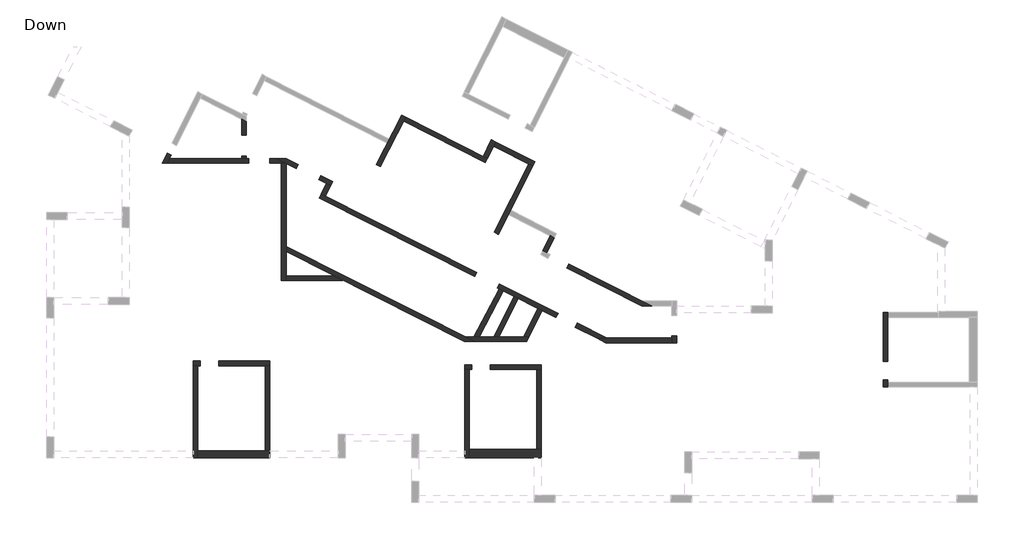
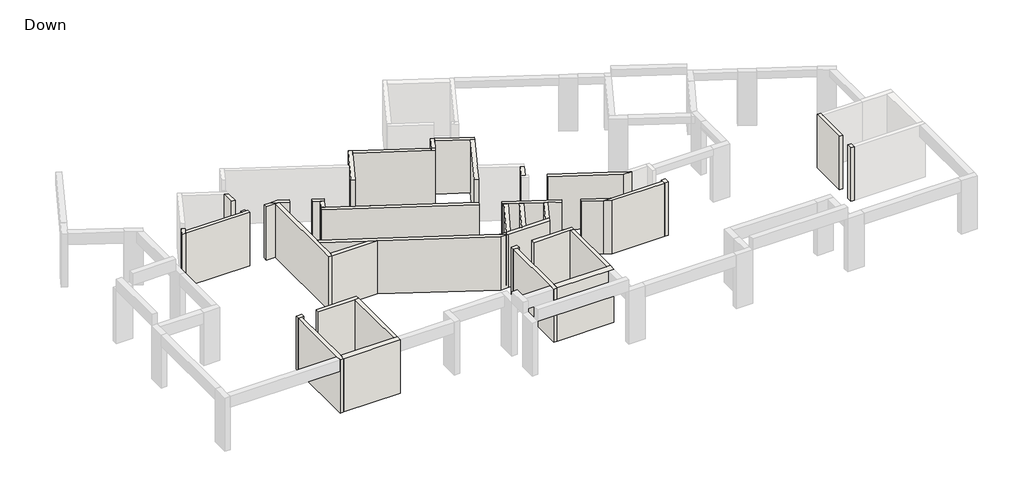
# One storey, part 1 of 3: 39 walls.
"""IFC4 building model written with IfcOpenShell, lengths in millimetres."""

from ifc_helpers import new_model, si_unit, origin, origin_with_axes, place, context, project, spatial, polyline, outline, extrude, faceted_brep, element, save

model = new_model("IFC4")

# Units and contexts
model_context = context("Model", 3, world=origin())
ifc_project = project(units=[si_unit("LENGTHUNIT", "METRE", prefix="MILLI")], contexts=[model_context])

# Site, building, storey
site = spatial("IfcSite", under=ifc_project)
building = spatial("IfcBuilding", under=site)
storey = spatial("IfcBuildingStorey", under=building, Name="Down", Elevation=0.0)

# Walls
placement = place(None, origin())
element("IfcWall", 1, ObjectType="20", at=placement, inside=storey, context=model_context, shape_type="Brep", body=[
    faceted_brep([(-10046.1154665, -6780.8119163, 0.0), (-10046.1154665, -6580.8119163, 0.0), (-10046.1154665, -5543.6743788, 0.0), (-10046.1154665, -5319.6317102, 0.0), (-10046.1154665, -1741.3845051, 0.0), (-10046.1154665, -1741.3845051, 3080.0), (-10046.1154665, -5319.6317102, 3080.0), (-10046.1154665, -5543.6743788, 3080.0), (-10046.1154665, -6580.8119163, 3080.0), (-10046.1154665, -6780.8119163, 3080.0), (-10246.1154665, -6780.8119163, 0.0), (-10246.1154665, -6780.8119163, 2780.0), (-10246.1154665, -6780.8119163, 3080.0), (-10246.1154665, -1726.4993482, 3080.0), (-10246.1154665, -1726.4993482, 2780.0), (-10246.1154665, -1726.4993482, 0.0), (-10075.8857802, -1726.4993482, 0.0), (-10075.8857802, -1726.4993482, 3080.0)], [[[0, 1, 2, 3, 4, 5, 6, 7, 8, 9]], [[10, 11, 12, 13, 14, 15]], [[4, 3, 2, 1, 0, 10, 15, 16]], [[9, 8, 7, 6, 5, 17, 13, 12]], [[5, 4, 16, 17]], [[16, 15, 14, 13, 17]], [[0, 9, 12, 11, 10]]]),
])
element("IfcWall", 2, ObjectType="20", at=placement, inside=storey, context=model_context, shape_type="Brep", body=[
    faceted_brep([(-10475.8857802, -1526.4993482, 0.0), (-10748.7939096, -1526.4993482, 0.0), (-10748.7939096, -1526.4993482, 2780.0), (-10748.7939096, -1526.4993482, 3080.0), (-10475.8857802, -1526.4993482, 3080.0), (-10075.8857802, -1726.4993482, 0.0), (-10075.8857802, -1726.4993482, 3080.0), (-10246.1154665, -1726.4993482, 3080.0), (-10748.7939096, -1726.4993482, 3080.0), (-10748.7939096, -1726.4993482, 2780.0), (-10748.7939096, -1726.4993482, 0.0), (-10246.1154665, -1726.4993482, 0.0)], [[[0, 1, 2, 3, 4]], [[5, 6, 7, 8, 9, 10, 11]], [[1, 0, 5, 11, 10]], [[3, 2, 1, 10, 9, 8]], [[4, 3, 8, 7, 6]], [[0, 4, 6, 5]]]),
])
element("IfcWall", 3, ObjectType="20", at=placement, inside=storey, context=model_context, shape_type="Brep", body=[
    faceted_brep([(-11648.323755, -1526.4993482, 0.0), (-11760.5135249, -1526.4993482, 0.0), (-11960.5135249, -1526.4993482, 0.0), (-15053.2787931, -1526.4993482, 0.0), (-15053.2787931, -1526.4993482, 2780.0), (-15053.2787931, -1526.4993482, 3080.0), (-11960.5135249, -1526.4993482, 3080.0), (-11760.5135249, -1526.4993482, 3080.0), (-11648.323755, -1526.4993482, 3080.0), (-11648.323755, -1526.4993482, 2780.0), (-11648.323755, -1726.4993482, 0.0), (-11648.323755, -1726.4993482, 2780.0), (-11648.323755, -1726.4993482, 3080.0), (-15153.2787931, -1726.4993482, 3080.0), (-15153.2787931, -1726.4993482, 0.0)], [[[0, 1, 2, 3, 4, 5, 6, 7, 8, 9]], [[10, 11, 12, 13, 14]], [[3, 2, 1, 0, 10, 14]], [[8, 7, 6, 5, 13, 12]], [[0, 9, 8, 12, 11, 10]], [[5, 4, 3, 14, 13]]]),
])
element("IfcWall", 4, ObjectType="20", at=placement, inside=storey, context=model_context, shape_type="Brep", body=[
    faceted_brep([(-15153.2787931, -1726.4993482, 0.0), (-15053.2787931, -1526.4993482, 0.0), (-14980.4135975, -1380.768957, 0.0), (-14980.4135975, -1380.768957, 2780.0), (-14980.4135975, -1380.768957, 3080.0), (-15053.2787931, -1526.4993482, 3080.0), (-15153.2787931, -1726.4993482, 3080.0), (-15376.8855909, -1726.4993482, 0.0), (-15376.8855909, -1726.4993482, 2780.0), (-15376.8855909, -1726.4993482, 3080.0), (-15159.2990357, -1291.3262379, 3080.0), (-15159.2990357, -1291.3262379, 2780.0), (-15159.2990357, -1291.3262379, 0.0)], [[[0, 1, 2, 3, 4, 5, 6]], [[7, 8, 9, 10, 11, 12]], [[2, 1, 0, 7, 12]], [[4, 3, 2, 12, 11, 10]], [[6, 5, 4, 10, 9]], [[0, 6, 9, 8, 7]]]),
])
element("IfcWall", 5, ObjectType="20", at=placement, inside=storey, context=model_context, shape_type="Brep", body=[
    faceted_brep([(-11960.5135249, 170.863779, 0.0), (-11960.5135249, -518.38158, 0.0), (-11960.5135249, -518.38158, 2780.0), (-11960.5135249, -518.38158, 3080.0), (-11960.5135249, 170.863779, 3080.0), (-11960.5135249, 170.863779, 2780.0), (-11760.5135249, 69.5479895, 0.0), (-11760.5135249, 69.5479895, 3080.0), (-11760.5135249, -518.38158, 3080.0), (-11760.5135249, -518.38158, 2780.0), (-11760.5135249, -518.38158, 0.0)], [[[0, 1, 2, 3, 4, 5]], [[6, 7, 8, 9, 10]], [[1, 0, 6, 10]], [[3, 2, 1, 10, 9, 8]], [[4, 3, 8, 7]], [[0, 5, 4, 7, 6]]]),
])
element("IfcWall", 6, ObjectType="20", at=placement, inside=storey, context=model_context, shape_type="Brep", body=[
    faceted_brep([(-11960.5135249, -1425.9636596, 0.0), (-11960.5135249, -1526.4993482, 0.0), (-11960.5135249, -1526.4993482, 2780.0), (-11960.5135249, -1526.4993482, 3080.0), (-11960.5135249, -1425.9636596, 3080.0), (-11960.5135249, -1425.9636596, 2780.0), (-11760.5135249, -1425.9636596, 0.0), (-11760.5135249, -1425.9636596, 2780.0), (-11760.5135249, -1425.9636596, 3080.0), (-11760.5135249, -1526.4993482, 3080.0), (-11760.5135249, -1526.4993482, 2780.0), (-11760.5135249, -1526.4993482, 0.0)], [[[0, 1, 2, 3, 4, 5]], [[6, 7, 8, 9, 10, 11]], [[1, 0, 6, 11]], [[4, 3, 9, 8]], [[0, 5, 4, 8, 7, 6]], [[3, 2, 1, 11, 10, 9]]]),
])
element("IfcWall", 7, ObjectType="20", at=placement, inside=storey, context=model_context, shape_type="Brep", body=[
    faceted_brep([(-5982.9078517, -1881.7028715, 0.0), (-4985.9127135, 79.4194333, 0.0), (-4895.2767918, 257.7032792, 0.0), (-4895.2767918, 257.7032792, 3080.0), (-4985.9127135, 79.4194333, 3080.0), (-5982.9078517, -1881.7028715, 3080.0), (-6161.1916976, -1791.0669498, 0.0), (-6161.1916976, -1791.0669498, 2780.0), (-6161.1916976, -1791.0669498, 3080.0), (-5688.8111915, -861.8789214, 3080.0), (-5598.1752698, -683.5950755, 3080.0), (-5073.5606377, 348.3392009, 3080.0), (-5073.5606377, 348.3392009, 2780.0), (-5073.5606377, 348.3392009, 0.0), (-5598.1752698, -683.5950755, 0.0), (-5688.8111915, -861.8789214, 0.0)], [[[0, 1, 2, 3, 4, 5]], [[6, 7, 8, 9, 10, 11, 12, 13, 14, 15]], [[2, 1, 0, 6, 15, 14, 13]], [[5, 4, 3, 11, 10, 9, 8]], [[0, 5, 8, 7, 6]], [[3, 2, 13, 12, 11]]]),
])
element("IfcWall", 8, ObjectType="20", at=placement, inside=storey, context=model_context, shape_type="Brep", body=[
    faceted_brep([(-4985.9127135, 79.4194333, 0.0), (-1478.212729, -1703.8246929, 0.0), (-1478.212729, -1703.8246929, 3080.0), (-4985.9127135, 79.4194333, 3080.0), (-4895.2767918, 257.7032792, 0.0), (-4895.2767918, 257.7032792, 3080.0), (-1565.8606533, -1434.9049253, 3080.0), (-1387.5768074, -1525.540847, 3080.0), (-1387.5768074, -1525.540847, 0.0), (-1565.8606533, -1434.9049253, 0.0)], [[[0, 1, 2, 3]], [[4, 5, 6, 7, 8, 9]], [[1, 0, 4, 9, 8]], [[3, 2, 7, 6, 5]], [[0, 3, 5, 4]], [[2, 1, 8, 7]]]),
])
element("IfcWall", 9, ObjectType="20", at=placement, inside=storey, context=model_context, shape_type="Brep", body=[
    faceted_brep([(-1387.5768074, -1525.540847, 0.0), (-1115.669538, -990.6902841, 0.0), (-1025.0331208, -812.4054634, 0.0), (-1025.0331208, -812.4054634, 3080.0), (-1115.669538, -990.6902841, 3080.0), (-1387.5768074, -1525.540847, 3080.0), (-1565.8606533, -1434.9049253, 0.0), (-1565.8606533, -1434.9049253, 2780.0), (-1565.8606533, -1434.9049253, 3080.0), (-1203.6166871, -722.3591018, 3080.0), (-1203.6166871, -722.3591018, 2780.0), (-1203.6166871, -722.3591018, 0.0)], [[[0, 1, 2, 3, 4, 5]], [[6, 7, 8, 9, 10, 11]], [[2, 1, 0, 6, 11]], [[5, 4, 3, 9, 8]], [[0, 5, 8, 7, 6]], [[3, 2, 11, 10, 9]]]),
])
element("IfcWall", 10, ObjectType="20", at=placement, inside=storey, context=model_context, shape_type="Brep", body=[
    faceted_brep([(-1115.669538, -990.6902841, 0.0), (402.8730243, -1756.3779423, 0.0), (581.4556142, -1846.4238115, 0.0), (581.4556142, -1846.4238115, 3080.0), (402.8730243, -1756.3779423, 3080.0), (-1115.669538, -990.6902841, 3080.0), (-1025.0331208, -812.4054634, 0.0), (-1025.0331208, -812.4054634, 3080.0), (54.7682985, -1356.8687143, 3080.0), (671.5014835, -1667.8412216, 3080.0), (671.5014835, -1667.8412216, 2780.0), (671.5014835, -1667.8412216, 0.0)], [[[0, 1, 2, 3, 4, 5]], [[6, 7, 8, 9, 10, 11]], [[2, 1, 0, 6, 11]], [[5, 4, 3, 9, 8, 7]], [[0, 5, 7, 6]], [[3, 2, 11, 10, 9]]]),
])
element("IfcWall", 11, ObjectType="20", at=placement, inside=storey, context=model_context, shape_type="Brep", body=[
    faceted_brep([(402.8730243, -1756.3779423, 0.0), (-1082.8838189, -4702.990676, 0.0), (-1082.8838189, -4702.990676, 3080.0), (402.8730243, -1756.3779423, 3080.0), (581.4556142, -1846.4238115, 0.0), (581.4556142, -1846.4238115, 3080.0), (-382.0351871, -3757.2575237, 3080.0), (-472.0818656, -3935.8417186, 3080.0), (-904.301229, -4793.0365453, 3080.0), (-904.301229, -4793.0365453, 2780.0), (-904.301229, -4793.0365453, 0.0), (-472.0818656, -3935.8417186, 0.0), (-382.0351871, -3757.2575237, 0.0)], [[[0, 1, 2, 3]], [[4, 5, 6, 7, 8, 9, 10, 11, 12]], [[1, 0, 4, 12, 11, 10]], [[2, 1, 10, 9, 8]], [[3, 2, 8, 7, 6, 5]], [[0, 3, 5, 4]]]),
])
element("IfcWall", 12, ObjectType="20", at=placement, inside=storey, context=model_context, shape_type="Brep", body=[
    faceted_brep([(1327.1276693, -4852.636386, 0.0), (1001.0372857, -5493.9474736, 0.0), (1001.0372857, -5493.9474736, 3080.0), (1327.1276693, -4852.636386, 3080.0), (1327.1276693, -4852.636386, 2780.0), (1505.3269714, -4943.4385782, 0.0), (1505.3269714, -4943.4385782, 3080.0), (1179.5082357, -5584.2154251, 3080.0), (1179.5082357, -5584.2154251, 2780.0), (1179.5082357, -5584.2154251, 0.0)], [[[0, 1, 2, 3, 4]], [[5, 6, 7, 8, 9]], [[1, 0, 5, 9]], [[3, 2, 7, 6]], [[0, 4, 3, 6, 5]], [[2, 1, 9, 8, 7]]]),
])
element("IfcWall", 13, ObjectType="20", at=placement, inside=storey, context=model_context, shape_type="Brep", body=[
    faceted_brep([(2035.1126004, -6241.094009, 0.0), (5265.429403, -7874.9401934, 0.0), (5265.429403, -7874.9401934, 2780.0), (5265.429403, -7874.9401934, 3080.0), (2035.1126004, -6241.094009, 3080.0), (2035.1126004, -6241.094009, 2780.0), (2125.3803454, -6062.6234674, 0.0), (2125.3803454, -6062.6234674, 2780.0), (2125.3803454, -6062.6234674, 3080.0), (5313.1307352, -7674.9401934, 3080.0), (5708.5555718, -7874.9401934, 3080.0), (5708.5555718, -7874.9401934, 0.0), (5313.1307352, -7674.9401934, 0.0), (2077.6096629, -6157.072039, 3080.0)], [[[0, 1, 2, 3, 4, 5]], [[6, 7, 8, 9, 10, 11, 12]], [[1, 0, 6, 12, 11]], [[4, 3, 10, 9, 8, 13]], [[0, 5, 4, 13, 8, 7, 6]], [[3, 2, 1, 11, 10]]]),
])
element("IfcWall", 14, ObjectType="20", at=placement, inside=storey, context=model_context, shape_type="Brep", body=[
    faceted_brep([(6570.8726693, -9167.2116828, 0.0), (6570.8726693, -9268.8187486, 0.0), (6570.8726693, -9468.8187486, 0.0), (6570.8726693, -9468.8187486, 3080.0), (6570.8726693, -9268.8187486, 3080.0), (6570.8726693, -9167.2116828, 3080.0), (6570.8726693, -9167.2116828, 2780.0), (6770.8726693, -9167.2116828, 0.0), (6770.8726693, -9167.2116828, 2780.0), (6770.8726693, -9167.2116828, 3080.0), (6770.8726693, -9468.8187486, 3080.0), (6770.8726693, -9468.8187486, 2780.0), (6770.8726693, -9468.8187486, 0.0)], [[[0, 1, 2, 3, 4, 5, 6]], [[7, 8, 9, 10, 11, 12]], [[2, 1, 0, 7, 12]], [[5, 4, 3, 10, 9]], [[0, 6, 5, 9, 8, 7]], [[3, 2, 12, 11, 10]]]),
])
element("IfcWall", 15, ObjectType="20", at=placement, inside=storey, context=model_context, shape_type="Brep", body=[
    faceted_brep([(6570.8726693, -9268.8187486, 0.0), (3765.4759744, -9268.8187486, 0.0), (3322.4500467, -9268.8187486, 0.0), (3322.4500467, -9268.8187486, 3080.0), (3765.4759744, -9268.8187486, 3080.0), (6570.8726693, -9268.8187486, 3080.0), (6570.8726693, -9268.8187486, 2780.0), (6570.8726693, -9468.8187486, 0.0), (6570.8726693, -9468.8187486, 3080.0), (3717.7625467, -9468.8187486, 3080.0), (3717.7625467, -9468.8187486, 2780.0), (3717.7625467, -9468.8187486, 0.0)], [[[0, 1, 2, 3, 4, 5, 6]], [[7, 8, 9, 10, 11]], [[2, 1, 0, 7, 11]], [[5, 4, 3, 9, 8]], [[0, 6, 5, 8, 7]], [[3, 2, 11, 10, 9]]]),
])
element("IfcWall", 16, ObjectType="20", at=placement, inside=storey, context=model_context, shape_type="Brep", body=[
    faceted_brep([(3765.4759744, -9268.8187486, 0.0), (2487.4451637, -8622.2260855, 0.0), (2487.4451637, -8622.2260855, 2780.0), (2487.4451637, -8622.2260855, 3080.0), (3765.4759744, -9268.8187486, 3080.0), (3765.4759744, -9268.8187486, 2780.0), (3322.4500467, -9268.8187486, 0.0), (3322.4500467, -9268.8187486, 3080.0), (2397.1569943, -8800.6862953, 3080.0), (2397.1569943, -8800.6862953, 2780.0), (2397.1569943, -8800.6862953, 0.0)], [[[0, 1, 2, 3, 4, 5]], [[6, 7, 8, 9, 10]], [[1, 0, 6, 10]], [[3, 2, 1, 10, 9, 8]], [[4, 3, 8, 7]], [[0, 5, 4, 7, 6]]]),
])
element("IfcWall", 17, ObjectType="20", at=placement, inside=storey, context=model_context, shape_type="Brep", body=[
    faceted_brep([(1666.9910125, -8207.1346573, 0.0), (-860.136602, -6928.58788, 0.0), (-860.136602, -6928.58788, 2780.0), (-860.136602, -6928.58788, 3080.0), (1666.9910125, -8207.1346573, 3080.0), (1666.9910125, -8207.1346573, 2780.0), (1576.7028432, -8385.594867, 0.0), (1576.7028432, -8385.594867, 2780.0), (1576.7028432, -8385.594867, 3080.0), (979.8740908, -8083.6419805, 3080.0), (979.5487996, -8083.4774063, 3080.0), (801.086592, -7993.1882261, 3080.0), (-42.8153908, -7566.2338633, 3080.0), (-221.2756006, -7475.9456939, 3080.0), (-696.8020222, -7235.3631565, 3080.0), (-875.2761926, -7145.067924, 3080.0), (-950.4247713, -7107.0480897, 3080.0), (-950.4247713, -7107.0480897, 2780.0), (-950.4247713, -7107.0480897, 0.0), (-875.2761926, -7145.067924, 0.0), (-696.8020222, -7235.3631565, 0.0), (-221.2756006, -7475.9456939, 0.0), (-42.8153908, -7566.2338633, 0.0), (801.086592, -7993.1882261, 0.0), (979.5487996, -8083.4774063, 0.0)], [[[0, 1, 2, 3, 4, 5]], [[6, 7, 8, 9, 10, 11, 12, 13, 14, 15, 16, 17, 18, 19, 20, 21, 22, 23, 24]], [[1, 0, 6, 24, 23, 22, 21, 20, 19, 18]], [[3, 2, 1, 18, 17, 16]], [[4, 3, 16, 15, 14, 13, 12, 11, 10, 9, 8]], [[0, 5, 4, 8, 7, 6]]]),
])
element("IfcWall", 18, ObjectType="20", at=placement, inside=storey, context=model_context, shape_type="Brep", body=[
    faceted_brep([(-1838.1570872, -6436.8740342, 0.0), (-8353.2474072, -3147.7022221, 0.0), (-8531.7861682, -3057.5661486, 0.0), (-8531.7861682, -3057.5661486, 3080.0), (-8353.2474072, -3147.7022221, 3080.0), (-1838.1570872, -6436.8740342, 3080.0), (-1838.1570872, -6436.8740342, 2780.0), (-1928.2924837, -6615.4114541, 0.0), (-1928.2924837, -6615.4114541, 3080.0), (-8621.2295591, -3236.4529305, 3080.0), (-8621.2295591, -3236.4529305, 0.0), (-1927.470094, -6613.7824899, 3080.0)], [[[0, 1, 2, 3, 4, 5, 6]], [[7, 8, 9, 10]], [[2, 1, 0, 7, 10]], [[5, 4, 3, 9, 8, 11]], [[0, 6, 5, 11, 8, 7]], [[3, 2, 10, 9]]]),
])
element("IfcWall", 19, ObjectType="20", at=placement, inside=storey, context=model_context, shape_type="Brep", body=[
    faceted_brep([(-8353.2474072, -3147.7022221, 0.0), (-8129.2939322, -2699.7952722, 0.0), (-8129.2939322, -2699.7952722, 3080.0), (-8353.2474072, -3147.7022221, 3080.0), (-8353.2474072, -3147.7022221, 2780.0), (-8531.7861682, -3057.5661486, 0.0), (-8531.7861682, -3057.5661486, 3080.0), (-8308.1793704, -2610.3525531, 3080.0), (-8308.1793704, -2610.3525531, 0.0)], [[[0, 1, 2, 3, 4]], [[5, 6, 7, 8]], [[1, 0, 5, 8]], [[3, 2, 7, 6]], [[0, 4, 3, 6, 5]], [[2, 1, 8, 7]]]),
])
element("IfcWall", 20, ObjectType="20", at=placement, inside=storey, context=model_context, shape_type="Brep", body=[
    faceted_brep([(-8039.8512131, -2520.909834, 0.0), (-8558.6189839, -2261.5259486, 0.0), (-8558.6189839, -2261.5259486, 2780.0), (-8558.6189839, -2261.5259486, 3080.0), (-8039.8512131, -2520.909834, 3080.0), (-8039.8512131, -2520.909834, 2780.0), (-8129.2939322, -2699.7952722, 0.0), (-8129.2939322, -2699.7952722, 3080.0), (-8308.1793704, -2610.3525531, 3080.0), (-8648.061703, -2440.4113868, 3080.0), (-8648.061703, -2440.4113868, 2780.0), (-8648.061703, -2440.4113868, 0.0), (-8308.1793704, -2610.3525531, 0.0)], [[[0, 1, 2, 3, 4, 5]], [[6, 7, 8, 9, 10, 11, 12]], [[1, 0, 6, 12, 11]], [[3, 2, 1, 11, 10, 9]], [[4, 3, 9, 8, 7]], [[0, 5, 4, 7, 6]]]),
])
element("IfcWall", 21, ObjectType="20", at=placement, inside=storey, context=model_context, shape_type="Brep", body=[
    faceted_brep([(-9512.4602897, -1784.6052957, 0.0), (-10028.6721847, -1526.4993482, 0.0), (-10028.6721847, -1526.4993482, 2780.0), (-10028.6721847, -1526.4993482, 3080.0), (-9512.4602897, -1784.6052957, 3080.0), (-9512.4602897, -1784.6052957, 2780.0), (-9601.9030088, -1963.4907339, 0.0), (-9601.9030088, -1963.4907339, 2780.0), (-9601.9030088, -1963.4907339, 3080.0), (-10046.1154665, -1741.3845051, 3080.0), (-10075.8857802, -1726.4993482, 3080.0), (-10475.8857802, -1526.4993482, 3080.0), (-10475.8857802, -1526.4993482, 0.0), (-10075.8857802, -1726.4993482, 0.0), (-10046.1154665, -1741.3845051, 0.0)], [[[0, 1, 2, 3, 4, 5]], [[6, 7, 8, 9, 10, 11, 12, 13, 14]], [[1, 0, 6, 14, 13, 12]], [[4, 3, 11, 10, 9, 8]], [[0, 5, 4, 8, 7, 6]], [[3, 2, 1, 12, 11]]]),
])
element("IfcWall", 22, ObjectType="20", at=placement, inside=storey, context=model_context, shape_type="Brep", body=[
    faceted_brep([(-10738.2112055, -10257.2302015, 0.0), (-12939.4136509, -10257.2302015, 0.0), (-12939.4136509, -10257.2302015, 2780.0), (-12939.4136509, -10257.2302015, 3080.0), (-10738.2112055, -10257.2302015, 3080.0), (-10738.2112055, -10257.2302015, 2780.0), (-10738.2112055, -10457.2302015, 0.0), (-10738.2112055, -10457.2302015, 3080.0), (-10938.2112055, -10457.2302015, 3080.0), (-12939.4136509, -10457.2302015, 3080.0), (-12939.4136509, -10457.2302015, 2780.0), (-12939.4136509, -10457.2302015, 0.0), (-10938.2112055, -10457.2302015, 0.0)], [[[0, 1, 2, 3, 4, 5]], [[6, 7, 8, 9, 10, 11, 12]], [[1, 0, 6, 12, 11]], [[3, 2, 1, 11, 10, 9]], [[4, 3, 9, 8, 7]], [[0, 5, 4, 7, 6]]]),
])
element("IfcWall", 23, ObjectType="20", at=placement, inside=storey, context=model_context, shape_type="Brep", body=[
    faceted_brep([(-13738.4078078, -10257.2302015, 0.0), (-14040.0148736, -10257.2302015, 0.0), (-14040.0148736, -10257.2302015, 2780.0), (-14040.0148736, -10257.2302015, 3080.0), (-13738.4078078, -10257.2302015, 3080.0), (-13738.4078078, -10257.2302015, 2780.0), (-13738.4078078, -10457.2302015, 0.0), (-13738.4078078, -10457.2302015, 2780.0), (-13738.4078078, -10457.2302015, 3080.0), (-13840.0148736, -10457.2302015, 3080.0), (-14040.0148736, -10457.2302015, 3080.0), (-14040.0148736, -10457.2302015, 0.0), (-13840.0148736, -10457.2302015, 0.0)], [[[0, 1, 2, 3, 4, 5]], [[6, 7, 8, 9, 10, 11, 12]], [[1, 0, 6, 12, 11]], [[4, 3, 10, 9, 8]], [[0, 5, 4, 8, 7, 6]], [[3, 2, 1, 11, 10]]]),
])
element("IfcWall", 24, ObjectType="20", at=placement, inside=storey, context=model_context, shape_type="Brep", body=[
    faceted_brep([(-14040.0148736, -10457.2302015, 0.0), (-14040.0148736, -14416.2328988, 0.0), (-14040.0148736, -14416.2328988, 3080.0), (-14040.0148736, -14116.2328988, 3080.0), (-14040.0148736, -10457.2302015, 3080.0), (-13840.0148736, -10457.2302015, 0.0), (-13840.0148736, -10457.2302015, 2780.0), (-13840.0148736, -10457.2302015, 3080.0), (-13840.0148736, -14116.2328988, 3080.0), (-13840.0148736, -14416.2328988, 3080.0), (-13840.0148736, -14416.2328988, 0.0), (-13840.0148736, -14116.2328988, 0.0)], [[[0, 1, 2, 3, 4]], [[5, 6, 7, 8, 9, 10, 11]], [[1, 0, 5, 11, 10]], [[4, 3, 2, 9, 8, 7]], [[0, 4, 7, 6, 5]], [[2, 1, 10, 9]]]),
])
element("IfcWall", 25, ObjectType="20", at=placement, inside=storey, context=model_context, shape_type="Brep", body=[
    faceted_brep([(-10738.2112055, -14116.2328988, 0.0), (-10738.2112055, -10457.2302015, 0.0), (-10738.2112055, -10457.2302015, 3080.0), (-10738.2112055, -14116.2328988, 3080.0), (-10738.2112055, -14116.2328988, 2780.0), (-10938.2112055, -14116.2328988, 0.0), (-10938.2112055, -14116.2328988, 2780.0), (-10938.2112055, -14116.2328988, 3080.0), (-10938.2112055, -10457.2302015, 3080.0), (-10938.2112055, -10457.2302015, 2780.0), (-10938.2112055, -10457.2302015, 0.0)], [[[0, 1, 2, 3, 4]], [[5, 6, 7, 8, 9, 10]], [[1, 0, 5, 10]], [[3, 2, 8, 7]], [[0, 4, 3, 7, 6, 5]], [[2, 1, 10, 9, 8]]]),
])
element("IfcWall", 26, ObjectType="20", at=placement, inside=storey, context=model_context, shape_type="Brep", body=[
    faceted_brep([(945.0940817, -10417.0421397, 0.0), (-1256.1083637, -10417.0421397, 0.0), (-1256.1083637, -10417.0421397, 2780.0), (-1256.1083637, -10417.0421397, 3080.0), (945.0940817, -10417.0421397, 3080.0), (945.0940817, -10417.0421397, 2780.0), (945.0940817, -10617.0421397, 0.0), (945.0940817, -10617.0421397, 3080.0), (745.0940817, -10617.0421397, 3080.0), (-1256.1083637, -10617.0421397, 3080.0), (-1256.1083637, -10617.0421397, 2780.0), (-1256.1083637, -10617.0421397, 0.0), (745.0940817, -10617.0421397, 0.0)], [[[0, 1, 2, 3, 4, 5]], [[6, 7, 8, 9, 10, 11, 12]], [[1, 0, 6, 12, 11]], [[3, 2, 1, 11, 10, 9]], [[4, 3, 9, 8, 7]], [[0, 5, 4, 7, 6]]]),
])
element("IfcWall", 27, ObjectType="20", at=placement, inside=storey, context=model_context, shape_type="Brep", body=[
    faceted_brep([(-2055.1025205, -10417.0421397, 0.0), (-2356.7095864, -10417.0421397, 0.0), (-2356.7095864, -10417.0421397, 2780.0), (-2356.7095864, -10417.0421397, 3080.0), (-2055.1025205, -10417.0421397, 3080.0), (-2055.1025205, -10417.0421397, 2780.0), (-2055.1025205, -10617.0421397, 0.0), (-2055.1025205, -10617.0421397, 2780.0), (-2055.1025205, -10617.0421397, 3080.0), (-2156.7095864, -10617.0421397, 3080.0), (-2356.7095864, -10617.0421397, 3080.0), (-2356.7095864, -10617.0421397, 0.0), (-2156.7095864, -10617.0421397, 0.0)], [[[0, 1, 2, 3, 4, 5]], [[6, 7, 8, 9, 10, 11, 12]], [[1, 0, 6, 12, 11]], [[4, 3, 10, 9, 8]], [[0, 5, 4, 8, 7, 6]], [[3, 2, 1, 11, 10]]]),
])
element("IfcWall", 28, ObjectType="20", at=placement, inside=storey, context=model_context, shape_type="Brep", body=[
    faceted_brep([(-2356.7095864, -10617.0421397, 0.0), (-2356.7095864, -14416.2328988, 0.0), (-2356.7095864, -14416.2328988, 2430.0), (-2356.7095864, -14416.2328988, 3080.0), (-2356.7095864, -14116.2328988, 3080.0), (-2356.7095864, -10617.0421397, 3080.0), (-2156.7095864, -10617.0421397, 0.0), (-2156.7095864, -10617.0421397, 2780.0), (-2156.7095864, -10617.0421397, 3080.0), (-2156.7095864, -14066.2328988, 3080.0), (-2156.7095864, -14416.2328988, 3080.0), (-2156.7095864, -14416.2328988, 0.0), (-2156.7095864, -14066.2328988, 0.0)], [[[0, 1, 2, 3, 4, 5]], [[6, 7, 8, 9, 10, 11, 12]], [[1, 0, 6, 12, 11]], [[5, 4, 3, 10, 9, 8]], [[0, 5, 8, 7, 6]], [[3, 2, 1, 11, 10]]]),
])
element("IfcWall", 29, ObjectType="20", at=placement, inside=storey, context=model_context, shape_type="Brep", body=[
    faceted_brep([(945.0940817, -14066.2328988, 0.0), (945.0940817, -10617.0421397, 0.0), (945.0940817, -10617.0421397, 3080.0), (945.0940817, -14066.2328988, 3080.0), (745.0940817, -14066.2328988, 0.0), (745.0940817, -14066.2328988, 2780.0), (745.0940817, -14066.2328988, 3080.0), (745.0940817, -10617.0421397, 3080.0), (745.0940817, -10617.0421397, 2780.0), (745.0940817, -10617.0421397, 0.0)], [[[0, 1, 2, 3]], [[4, 5, 6, 7, 8, 9]], [[1, 0, 4, 9]], [[3, 2, 7, 6]], [[0, 3, 6, 5, 4]], [[2, 1, 9, 8, 7]]]),
])
element("IfcWall", 30, ObjectType="20", at=placement, inside=storey, context=model_context, shape_type="Brep", body=[
    faceted_brep([(15670.9267875, -11066.8070624, 0.0), (15670.9267875, -11368.4141282, 0.0), (15670.9267875, -11368.4141282, 2780.0), (15670.9267875, -11368.4141282, 3080.0), (15670.9267875, -11066.8070624, 3080.0), (15670.9267875, -11066.8070624, 2780.0), (15870.9267875, -11066.8070624, 0.0), (15870.9267875, -11066.8070624, 2780.0), (15870.9267875, -11066.8070624, 3080.0), (15870.9267875, -11168.4141282, 3080.0), (15870.9267875, -11368.4141282, 3080.0), (15870.9267875, -11368.4141282, 0.0), (15870.9267875, -11168.4141282, 0.0)], [[[0, 1, 2, 3, 4, 5]], [[6, 7, 8, 9, 10, 11, 12]], [[1, 0, 6, 12, 11]], [[4, 3, 10, 9, 8]], [[0, 5, 4, 8, 7, 6]], [[3, 2, 1, 11, 10]]]),
])
element("IfcWall", 31, ObjectType="20", at=placement, inside=storey, context=model_context, shape_type="Brep", body=[
    faceted_brep([(15870.9267875, -10267.8129055, 0.0), (15870.9267875, -8367.1461487, 0.0), (15870.9267875, -8167.1461487, 0.0), (15870.9267875, -8167.1461487, 3080.0), (15870.9267875, -8367.1461487, 3080.0), (15870.9267875, -10267.8129055, 3080.0), (15870.9267875, -10267.8129055, 2780.0), (15670.9267875, -10267.8129055, 0.0), (15670.9267875, -10267.8129055, 2780.0), (15670.9267875, -10267.8129055, 3080.0), (15670.9267875, -8167.1461487, 3080.0), (15670.9267875, -8167.1461487, 2780.0), (15670.9267875, -8167.1461487, 0.0)], [[[0, 1, 2, 3, 4, 5, 6]], [[7, 8, 9, 10, 11, 12]], [[2, 1, 0, 7, 12]], [[5, 4, 3, 10, 9]], [[0, 6, 5, 9, 8, 7]], [[3, 2, 12, 11, 10]]]),
])
element("IfcWall", 32, ObjectType="20", at=placement, inside=storey, context=model_context, shape_type="Brep", body=[
    faceted_brep([(-10046.1154665, -6780.8119163, 0.0), (-7595.6314981, -6780.8119163, 0.0), (-7595.6314981, -6780.8119163, 2780.0), (-7595.6314981, -6780.8119163, 3080.0), (-10046.1154665, -6780.8119163, 3080.0), (-7991.7853443, -6580.8119163, 0.0), (-10046.1154665, -6580.8119163, 0.0), (-10046.1154665, -6580.8119163, 3080.0), (-7991.7853443, -6580.8119163, 3080.0)], [[[0, 1, 2, 3, 4]], [[5, 6, 7, 8]], [[1, 0, 6, 5]], [[4, 3, 8, 7]], [[0, 4, 7, 6]], [[3, 2, 1, 5, 8]]]),
])
element("IfcWall", 33, ObjectType="20", at=placement, inside=storey, context=model_context, shape_type="Brep", body=[
    faceted_brep([(-10046.1154665, -5543.6743788, 0.0), (-7991.7853443, -6580.8119163, 0.0), (-7595.6314981, -6780.8119163, 0.0), (-2368.5637573, -9419.7199019, 0.0), (-2368.5637573, -9419.7199019, 2780.0), (-2368.5637573, -9419.7199019, 3080.0), (-7595.6314981, -6780.8119163, 3080.0), (-7991.7853443, -6580.8119163, 3080.0), (-10046.1154665, -5543.6743788, 3080.0), (-1924.7869329, -9419.7199019, 0.0), (-2320.9407791, -9219.7199019, 0.0), (-10046.1154665, -5319.6317102, 0.0), (-10046.1154665, -5319.6317102, 3080.0), (-2320.9407791, -9219.7199019, 3080.0), (-1924.7869329, -9419.7199019, 3080.0)], [[[0, 1, 2, 3, 4, 5, 6, 7, 8]], [[9, 10, 11, 12, 13, 14]], [[3, 2, 1, 0, 11, 10, 9]], [[8, 7, 6, 5, 14, 13, 12]], [[5, 4, 3, 9, 14]], [[0, 8, 12, 11]]]),
])
element("IfcWall", 34, ObjectType="20", at=placement, inside=storey, context=model_context, shape_type="Brep", body=[
    faceted_brep([(-1924.7869329, -9419.7199019, 0.0), (311.4275518, -9419.7199019, 0.0), (311.4275518, -9419.7199019, 2780.0), (311.4275518, -9419.7199019, 3080.0), (-1924.7869329, -9419.7199019, 3080.0), (-2320.9407791, -9219.7199019, 0.0), (-2320.9407791, -9219.7199019, 3080.0), (-1957.7033115, -9219.7199019, 3080.0), (-1732.1185851, -9219.7199019, 3080.0), (-1103.5012868, -9219.7199019, 3080.0), (-879.361687, -9219.7199019, 3080.0), (187.820754, -9219.7199019, 3080.0), (411.4275518, -9219.7199019, 3080.0), (411.4275518, -9219.7199019, 0.0), (187.820754, -9219.7199019, 0.0), (-879.361687, -9219.7199019, 0.0), (-1103.5012868, -9219.7199019, 0.0), (-1732.1185851, -9219.7199019, 0.0), (-1957.7033115, -9219.7199019, 0.0)], [[[0, 1, 2, 3, 4]], [[5, 6, 7, 8, 9, 10, 11, 12, 13, 14, 15, 16, 17, 18]], [[1, 0, 5, 18, 17, 16, 15, 14, 13]], [[4, 3, 12, 11, 10, 9, 8, 7, 6]], [[0, 4, 6, 5]], [[3, 2, 1, 13, 12]]]),
])
element("IfcWall", 35, ObjectType="20", at=placement, inside=storey, context=model_context, shape_type="Brep", body=[
    faceted_brep([(411.4275518, -9219.7199019, 0.0), (979.5487996, -8083.4774063, 0.0), (979.5487996, -8083.4774063, 3080.0), (945.0940817, -8152.386842, 3080.0), (411.4275518, -9219.7199019, 3080.0), (187.820754, -9219.7199019, 0.0), (187.820754, -9219.7199019, 3080.0), (801.086592, -7993.1882261, 3080.0), (801.086592, -7993.1882261, 0.0)], [[[0, 1, 2, 3, 4]], [[5, 6, 7, 8]], [[1, 0, 5, 8]], [[4, 3, 2, 7, 6]], [[0, 4, 6, 5]], [[2, 1, 8, 7]]]),
])
element("IfcWall", 36, ObjectType="20", at=placement, inside=storey, context=model_context, shape_type="SweptSolid", body=[
    extrude(outline(polyline([(-42.8153908, -7566.2338633), (-879.361687, -9219.7199019), (-1103.5012868, -9219.7199019), (-221.2756006, -7475.9456939), (-42.8153908, -7566.2338633)])), origin_with_axes(), (0.0, 0.0, 1.0), 3080.0),
])
element("IfcWall", 37, ObjectType="20", at=placement, inside=storey, context=model_context, shape_type="SweptSolid", body=[
    extrude(outline(polyline([(-696.8020222, -7235.3631565), (-1732.1185851, -9219.7199019), (-1957.7033115, -9219.7199019), (-875.2761926, -7145.067924), (-696.8020222, -7235.3631565)])), origin_with_axes(), (0.0, 0.0, 1.0), 3080.0),
])
element("IfcWall", 38, ObjectType="30", at=placement, inside=storey, context=model_context, shape_type="Brep", body=[
    faceted_brep([(-13840.0148736, -14416.2328988, 0.0), (-10738.2112055, -14416.2328988, 0.0), (-10738.2112055, -14416.2328988, 2430.0), (-10738.2112055, -14416.2328988, 3080.0), (-13840.0148736, -14416.2328988, 3080.0), (-13840.0148736, -14116.2328988, 0.0), (-13840.0148736, -14116.2328988, 2780.0), (-13840.0148736, -14116.2328988, 3080.0), (-10938.2112055, -14116.2328988, 3080.0), (-10738.2112055, -14116.2328988, 3080.0), (-10738.2112055, -14116.2328988, 2430.0), (-10738.2112055, -14116.2328988, 0.0), (-10938.2112055, -14116.2328988, 0.0)], [[[0, 1, 2, 3, 4]], [[5, 6, 7, 8, 9, 10, 11, 12]], [[1, 0, 5, 12, 11]], [[4, 3, 9, 8, 7]], [[0, 4, 7, 6, 5]], [[3, 2, 1, 11, 10, 9]]]),
])
element("IfcWall", 39, ObjectType="35", at=placement, inside=storey, context=model_context, shape_type="Brep", body=[
    faceted_brep([(-2156.7095864, -14416.2328988, 0.0), (945.0940817, -14416.2328988, 0.0), (945.0940817, -14416.2328988, 3080.0), (-2156.7095864, -14416.2328988, 3080.0), (-2156.7095864, -14066.2328988, 0.0), (-2156.7095864, -14066.2328988, 2780.0), (-2156.7095864, -14066.2328988, 3080.0), (745.0940817, -14066.2328988, 3080.0), (945.0940817, -14066.2328988, 3080.0), (945.0940817, -14066.2328988, 0.0), (745.0940817, -14066.2328988, 0.0)], [[[0, 1, 2, 3]], [[4, 5, 6, 7, 8, 9, 10]], [[1, 0, 4, 10, 9]], [[3, 2, 8, 7, 6]], [[0, 3, 6, 5, 4]], [[2, 1, 9, 8]]]),
])

save(model, "model.ifc")

# Revit data of these elements
# Project information
#   Project Issue Date = "Issue Date"
#   Project Status = "Project Status"
#   Client Name = "לקוח"
#   Project Address = "Enter address here"
#   Project Name = "Project 045"
#   Project Number = "מספר פרויקט"
# Type "20"
#   Layers, outside or top first: 20 cm "Concrete" (function 1)
# Type "30"
#   Layers, outside or top first: 30 cm "Concrete" (function 1)
# Type "35"
#   Layers, outside or top first: 35 cm "Concrete" (function 1)
# Element 1 (IfcWall, "20")
#   Comments = ""
#   Mark = "W1"
#   SOFiSTiK_AMG_Comments = ""
#   Top Offset = 0 cm
#   Base Offset = 0 cm
#   wall height = 308 cm
#   SOFiSTiK_AMG_Scheduled = yes
#   SOFiSTiK_AMG_Adjusted = yes
#   Phase Created = New Construction
#   Base Constraint = Down
#   Top Constraint = Typical Floor
#   Materials on its faces: "Concrete"
# Element 2 (IfcWall, "20")
#   Comments = ""
#   Mark = "W2"
#   SOFiSTiK_AMG_Comments = ""
#   Top Offset = 0 cm
#   Base Offset = 0 cm
#   wall height = 308 cm
#   SOFiSTiK_AMG_Scheduled = yes
#   SOFiSTiK_AMG_Adjusted = yes
#   Phase Created = New Construction
#   Base Constraint = Down
#   Top Constraint = Typical Floor
#   Materials on its faces: "Concrete"
# Element 3 (IfcWall, "20")
#   Comments = ""
#   Mark = "W3"
#   SOFiSTiK_AMG_Comments = ""
#   Top Offset = 0 cm
#   Base Offset = 0 cm
#   wall height = 308 cm
#   SOFiSTiK_AMG_Scheduled = yes
#   SOFiSTiK_AMG_Adjusted = yes
#   Phase Created = New Construction
#   Base Constraint = Down
#   Top Constraint = Typical Floor
#   Materials on its faces: "Concrete"
# Element 4 (IfcWall, "20")
#   Comments = ""
#   Mark = "W4"
#   SOFiSTiK_AMG_Comments = ""
#   Top Offset = 0 cm
#   Base Offset = 0 cm
#   wall height = 308 cm
#   SOFiSTiK_AMG_Scheduled = yes
#   SOFiSTiK_AMG_Adjusted = yes
#   Phase Created = New Construction
#   Base Constraint = Down
#   Top Constraint = Typical Floor
#   Materials on its faces: "Concrete"
# Element 5 (IfcWall, "20")
#   Comments = ""
#   Mark = "W7"
#   SOFiSTiK_AMG_Comments = ""
#   Top Offset = 0 cm
#   Base Offset = 0 cm
#   wall height = 308 cm
#   SOFiSTiK_AMG_Scheduled = yes
#   SOFiSTiK_AMG_Adjusted = yes
#   Phase Created = New Construction
#   Base Constraint = Down
#   Top Constraint = Typical Floor
#   Materials on its faces: "Concrete"
# Element 6 (IfcWall, "20")
#   Comments = ""
#   Mark = "W8"
#   SOFiSTiK_AMG_Comments = "Too Short /"
#   Top Offset = 0 cm
#   Base Offset = 0 cm
#   wall height = 308 cm
#   SOFiSTiK_AMG_Scheduled = yes
#   SOFiSTiK_AMG_Adjusted = yes
#   Phase Created = New Construction
#   Base Constraint = Down
#   Top Constraint = Typical Floor
#   Materials on its faces: "Concrete"
# Element 7 (IfcWall, "20")
#   Comments = ""
#   Mark = "W12"
#   SOFiSTiK_AMG_Comments = ""
#   Top Offset = 0 cm
#   Base Offset = 0 cm
#   wall height = 308 cm
#   SOFiSTiK_AMG_Scheduled = yes
#   SOFiSTiK_AMG_Adjusted = yes
#   Phase Created = New Construction
#   Base Constraint = Down
#   Top Constraint = Typical Floor
#   Materials on its faces: "Concrete"
# Element 8 (IfcWall, "20")
#   Comments = ""
#   Mark = "W13"
#   SOFiSTiK_AMG_Comments = ""
#   Top Offset = 0 cm
#   Base Offset = 0 cm
#   wall height = 308 cm
#   SOFiSTiK_AMG_Scheduled = yes
#   SOFiSTiK_AMG_Adjusted = yes
#   Phase Created = New Construction
#   Base Constraint = Down
#   Top Constraint = Typical Floor
#   Materials on its faces: "Concrete"
# Element 9 (IfcWall, "20")
#   Comments = ""
#   Mark = "W14"
#   SOFiSTiK_AMG_Comments = ""
#   Top Offset = 0 cm
#   Base Offset = 0 cm
#   wall height = 308 cm
#   SOFiSTiK_AMG_Scheduled = yes
#   SOFiSTiK_AMG_Adjusted = yes
#   Phase Created = New Construction
#   Base Constraint = Down
#   Top Constraint = Typical Floor
#   Materials on its faces: "Concrete"
# Element 10 (IfcWall, "20")
#   Comments = ""
#   Mark = "W15"
#   SOFiSTiK_AMG_Comments = ""
#   Top Offset = 0 cm
#   Base Offset = 0 cm
#   wall height = 308 cm
#   SOFiSTiK_AMG_Scheduled = yes
#   SOFiSTiK_AMG_Adjusted = yes
#   Phase Created = New Construction
#   Base Constraint = Down
#   Top Constraint = Typical Floor
#   Materials on its faces: "Concrete"
# Element 11 (IfcWall, "20")
#   Comments = ""
#   Mark = "W16"
#   SOFiSTiK_AMG_Comments = ""
#   Top Offset = 0 cm
#   Base Offset = 0 cm
#   wall height = 308 cm
#   SOFiSTiK_AMG_Scheduled = yes
#   SOFiSTiK_AMG_Adjusted = yes
#   Phase Created = New Construction
#   Base Constraint = Down
#   Top Constraint = Typical Floor
#   Materials on its faces: "Concrete"
# Element 12 (IfcWall, "20")
#   Comments = ""
#   Mark = "W18"
#   SOFiSTiK_AMG_Comments = ""
#   Top Offset = 0 cm
#   Base Offset = 0 cm
#   wall height = 308 cm
#   SOFiSTiK_AMG_Scheduled = yes
#   SOFiSTiK_AMG_Adjusted = yes
#   Phase Created = New Construction
#   Base Constraint = Down
#   Top Constraint = Typical Floor
#   Materials on its faces: "Concrete"
# Element 13 (IfcWall, "20")
#   Comments = ""
#   Mark = "W20"
#   SOFiSTiK_AMG_Comments = ""
#   Top Offset = 0 cm
#   Base Offset = 0 cm
#   wall height = 308 cm
#   SOFiSTiK_AMG_Scheduled = yes
#   SOFiSTiK_AMG_Adjusted = yes
#   Phase Created = New Construction
#   Base Constraint = Down
#   Top Constraint = Typical Floor
#   Materials on its faces: "Concrete"
# Element 14 (IfcWall, "20")
#   Comments = ""
#   Mark = "W23"
#   SOFiSTiK_AMG_Comments = ""
#   Top Offset = 0 cm
#   Base Offset = 0 cm
#   wall height = 308 cm
#   SOFiSTiK_AMG_Scheduled = yes
#   SOFiSTiK_AMG_Adjusted = yes
#   Phase Created = New Construction
#   Base Constraint = Down
#   Top Constraint = Typical Floor
#   Materials on its faces: "Concrete"
# Element 15 (IfcWall, "20")
#   Comments = ""
#   Mark = "W24"
#   SOFiSTiK_AMG_Comments = ""
#   Top Offset = 0 cm
#   Base Offset = 0 cm
#   wall height = 308 cm
#   SOFiSTiK_AMG_Scheduled = yes
#   SOFiSTiK_AMG_Adjusted = yes
#   Phase Created = New Construction
#   Base Constraint = Down
#   Top Constraint = Typical Floor
#   Materials on its faces: "Concrete"
# Element 16 (IfcWall, "20")
#   Comments = ""
#   Mark = "W25"
#   SOFiSTiK_AMG_Comments = ""
#   Top Offset = 0 cm
#   Base Offset = 0 cm
#   wall height = 308 cm
#   SOFiSTiK_AMG_Scheduled = yes
#   SOFiSTiK_AMG_Adjusted = yes
#   Phase Created = New Construction
#   Base Constraint = Down
#   Top Constraint = Typical Floor
#   Materials on its faces: "Concrete"
# Element 17 (IfcWall, "20")
#   Comments = ""
#   Mark = "W26"
#   SOFiSTiK_AMG_Comments = ""
#   Top Offset = 0 cm
#   Base Offset = 0 cm
#   wall height = 308 cm
#   SOFiSTiK_AMG_Scheduled = yes
#   SOFiSTiK_AMG_Adjusted = yes
#   Phase Created = New Construction
#   Base Constraint = Down
#   Top Constraint = Typical Floor
#   Materials on its faces: "Concrete"
# Element 18 (IfcWall, "20")
#   Comments = ""
#   Mark = "W27"
#   SOFiSTiK_AMG_Comments = ""
#   Top Offset = 0 cm
#   Base Offset = 0 cm
#   wall height = 308 cm
#   SOFiSTiK_AMG_Scheduled = yes
#   SOFiSTiK_AMG_Adjusted = yes
#   Phase Created = New Construction
#   Base Constraint = Down
#   Top Constraint = Typical Floor
#   Materials on its faces: "Concrete"
# Element 19 (IfcWall, "20")
#   Comments = ""
#   Mark = "W28"
#   SOFiSTiK_AMG_Comments = ""
#   Top Offset = 0 cm
#   Base Offset = 0 cm
#   wall height = 308 cm
#   SOFiSTiK_AMG_Scheduled = yes
#   SOFiSTiK_AMG_Adjusted = yes
#   Phase Created = New Construction
#   Base Constraint = Down
#   Top Constraint = Typical Floor
#   Materials on its faces: "Concrete"
# Element 20 (IfcWall, "20")
#   Comments = ""
#   Mark = "W29"
#   SOFiSTiK_AMG_Comments = ""
#   Top Offset = 0 cm
#   Base Offset = 0 cm
#   wall height = 308 cm
#   SOFiSTiK_AMG_Scheduled = yes
#   SOFiSTiK_AMG_Adjusted = yes
#   Phase Created = New Construction
#   Base Constraint = Down
#   Top Constraint = Typical Floor
#   Materials on its faces: "Concrete"
# Element 21 (IfcWall, "20")
#   Comments = ""
#   Mark = "W30"
#   SOFiSTiK_AMG_Comments = ""
#   Top Offset = 0 cm
#   Base Offset = 0 cm
#   wall height = 308 cm
#   SOFiSTiK_AMG_Scheduled = yes
#   SOFiSTiK_AMG_Adjusted = yes
#   Phase Created = New Construction
#   Base Constraint = Down
#   Top Constraint = Typical Floor
#   Materials on its faces: "Concrete"
# Element 22 (IfcWall, "20")
#   Comments = ""
#   Mark = "W31"
#   SOFiSTiK_AMG_Comments = ""
#   Top Offset = 0 cm
#   Base Offset = 0 cm
#   wall height = 308 cm
#   SOFiSTiK_AMG_Scheduled = yes
#   SOFiSTiK_AMG_Adjusted = yes
#   Phase Created = New Construction
#   Base Constraint = Down
#   Top Constraint = Typical Floor
#   Materials on its faces: "Concrete"
# Element 23 (IfcWall, "20")
#   Comments = ""
#   Mark = "W32"
#   SOFiSTiK_AMG_Comments = ""
#   Top Offset = 0 cm
#   Base Offset = 0 cm
#   wall height = 308 cm
#   SOFiSTiK_AMG_Scheduled = yes
#   SOFiSTiK_AMG_Adjusted = yes
#   Phase Created = New Construction
#   Base Constraint = Down
#   Top Constraint = Typical Floor
#   Materials on its faces: "Concrete"
# Element 24 (IfcWall, "20")
#   Comments = ""
#   Mark = "W33"
#   SOFiSTiK_AMG_Comments = ""
#   Top Offset = 0 cm
#   Base Offset = 0 cm
#   wall height = 308 cm
#   SOFiSTiK_AMG_Scheduled = yes
#   SOFiSTiK_AMG_Adjusted = yes
#   Phase Created = New Construction
#   Base Constraint = Down
#   Top Constraint = Typical Floor
#   Materials on its faces: "Concrete"
# Element 25 (IfcWall, "20")
#   Comments = ""
#   Mark = "W34"
#   SOFiSTiK_AMG_Comments = ""
#   Top Offset = 0 cm
#   Base Offset = 0 cm
#   wall height = 308 cm
#   SOFiSTiK_AMG_Scheduled = yes
#   SOFiSTiK_AMG_Adjusted = yes
#   Phase Created = New Construction
#   Base Constraint = Down
#   Top Constraint = Typical Floor
#   Materials on its faces: "Concrete"
# Element 26 (IfcWall, "20")
#   Comments = ""
#   Mark = "W35"
#   SOFiSTiK_AMG_Comments = ""
#   Top Offset = 0 cm
#   Base Offset = 0 cm
#   wall height = 308 cm
#   SOFiSTiK_AMG_Scheduled = yes
#   SOFiSTiK_AMG_Adjusted = yes
#   Phase Created = New Construction
#   Base Constraint = Down
#   Top Constraint = Typical Floor
#   Materials on its faces: "Concrete"
# Element 27 (IfcWall, "20")
#   Comments = ""
#   Mark = "W36"
#   SOFiSTiK_AMG_Comments = ""
#   Top Offset = 0 cm
#   Base Offset = 0 cm
#   wall height = 308 cm
#   SOFiSTiK_AMG_Scheduled = yes
#   SOFiSTiK_AMG_Adjusted = yes
#   Phase Created = New Construction
#   Base Constraint = Down
#   Top Constraint = Typical Floor
#   Materials on its faces: "Concrete"
# Element 28 (IfcWall, "20")
#   Comments = ""
#   Mark = "W37"
#   SOFiSTiK_AMG_Comments = ""
#   Top Offset = 0 cm
#   Base Offset = 0 cm
#   wall height = 308 cm
#   SOFiSTiK_AMG_Scheduled = yes
#   SOFiSTiK_AMG_Adjusted = yes
#   Phase Created = New Construction
#   Base Constraint = Down
#   Top Constraint = Typical Floor
#   Materials on its faces: "Concrete"
# Element 29 (IfcWall, "20")
#   Comments = ""
#   Mark = "W38"
#   SOFiSTiK_AMG_Comments = ""
#   Top Offset = 0 cm
#   Base Offset = 0 cm
#   wall height = 308 cm
#   SOFiSTiK_AMG_Scheduled = yes
#   SOFiSTiK_AMG_Adjusted = yes
#   Phase Created = New Construction
#   Base Constraint = Down
#   Top Constraint = Typical Floor
#   Materials on its faces: "Concrete"
# Element 30 (IfcWall, "20")
#   Comments = ""
#   Mark = "W39"
#   SOFiSTiK_AMG_Comments = ""
#   Top Offset = 0 cm
#   Base Offset = 0 cm
#   wall height = 308 cm
#   SOFiSTiK_AMG_Scheduled = yes
#   SOFiSTiK_AMG_Adjusted = yes
#   Phase Created = New Construction
#   Base Constraint = Down
#   Top Constraint = Typical Floor
#   Materials on its faces: "Concrete"
# Element 31 (IfcWall, "20")
#   Comments = ""
#   Mark = "W41"
#   SOFiSTiK_AMG_Comments = ""
#   Top Offset = 0 cm
#   Base Offset = 0 cm
#   wall height = 308 cm
#   SOFiSTiK_AMG_Scheduled = yes
#   SOFiSTiK_AMG_Adjusted = yes
#   Phase Created = New Construction
#   Base Constraint = Down
#   Top Constraint = Typical Floor
#   Materials on its faces: "Concrete"
# Element 32 (IfcWall, "20")
#   Comments = ""
#   Mark = "W51"
#   SOFiSTiK_AMG_Comments = ""
#   Top Offset = 0 cm
#   Base Offset = 0 cm
#   wall height = 308 cm
#   SOFiSTiK_AMG_Scheduled = yes
#   SOFiSTiK_AMG_Adjusted = yes
#   Phase Created = New Construction
#   Base Constraint = Down
#   Top Constraint = Typical Floor
#   Materials on its faces: "Concrete"
# Element 33 (IfcWall, "20")
#   Comments = ""
#   Mark = "W52"
#   SOFiSTiK_AMG_Comments = ""
#   Top Offset = 0 cm
#   Base Offset = 0 cm
#   wall height = 308 cm
#   SOFiSTiK_AMG_Scheduled = yes
#   SOFiSTiK_AMG_Adjusted = yes
#   Phase Created = New Construction
#   Base Constraint = Down
#   Top Constraint = Typical Floor
#   Materials on its faces: "Concrete"
# Element 34 (IfcWall, "20")
#   Comments = ""
#   Mark = "W53"
#   SOFiSTiK_AMG_Comments = ""
#   Top Offset = 0 cm
#   Base Offset = 0 cm
#   wall height = 308 cm
#   SOFiSTiK_AMG_Scheduled = yes
#   SOFiSTiK_AMG_Adjusted = yes
#   Phase Created = New Construction
#   Base Constraint = Down
#   Top Constraint = Typical Floor
#   Materials on its faces: "Concrete"
# Element 35 (IfcWall, "20")
#   Comments = ""
#   Mark = "W54"
#   SOFiSTiK_AMG_Comments = ""
#   Top Offset = 0 cm
#   Base Offset = 0 cm
#   wall height = 308 cm
#   SOFiSTiK_AMG_Scheduled = yes
#   SOFiSTiK_AMG_Adjusted = yes
#   Phase Created = New Construction
#   Base Constraint = Down
#   Top Constraint = Typical Floor
#   Materials on its faces: "Concrete"
# Element 36 (IfcWall, "20")
#   Comments = ""
#   Mark = "W55"
#   SOFiSTiK_AMG_Comments = ""
#   Top Offset = 0 cm
#   Base Offset = 0 cm
#   wall height = 308 cm
#   SOFiSTiK_AMG_Scheduled = yes
#   SOFiSTiK_AMG_Adjusted = yes
#   Phase Created = New Construction
#   Base Constraint = Down
#   Top Constraint = Typical Floor
#   Materials on its faces: "Concrete"
# Element 37 (IfcWall, "20")
#   Comments = ""
#   Mark = "W56"
#   SOFiSTiK_AMG_Comments = ""
#   Top Offset = 0 cm
#   Base Offset = 0 cm
#   wall height = 308 cm
#   SOFiSTiK_AMG_Scheduled = yes
#   SOFiSTiK_AMG_Adjusted = yes
#   Phase Created = New Construction
#   Base Constraint = Down
#   Top Constraint = Typical Floor
#   Materials on its faces: "Concrete"
# Element 38 (IfcWall, "30")
#   Comments = ""
#   Mark = "W57"
#   SOFiSTiK_AMG_Comments = ""
#   Top Offset = 0 cm
#   Base Offset = 0 cm
#   wall height = 308 cm
#   SOFiSTiK_AMG_Scheduled = yes
#   SOFiSTiK_AMG_Adjusted = yes
#   Phase Created = New Construction
#   Base Constraint = Down
#   Top Constraint = Typical Floor
#   Materials on its faces: "Concrete"
# Element 39 (IfcWall, "35")
#   Comments = ""
#   Mark = "W58"
#   SOFiSTiK_AMG_Comments = ""
#   Top Offset = 0 cm
#   Base Offset = 0 cm
#   wall height = 308 cm
#   SOFiSTiK_AMG_Scheduled = yes
#   SOFiSTiK_AMG_Adjusted = yes
#   Phase Created = New Construction
#   Base Constraint = Down
#   Top Constraint = Typical Floor
#   Materials on its faces: "Concrete"
# Materials
#   "Concrete": class "Concrete", colour RGB 192 192 192, transparency 0, Keynote = "01000", Description = "Cast-in-place concrete", Cost = 0
